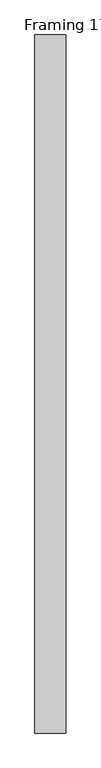
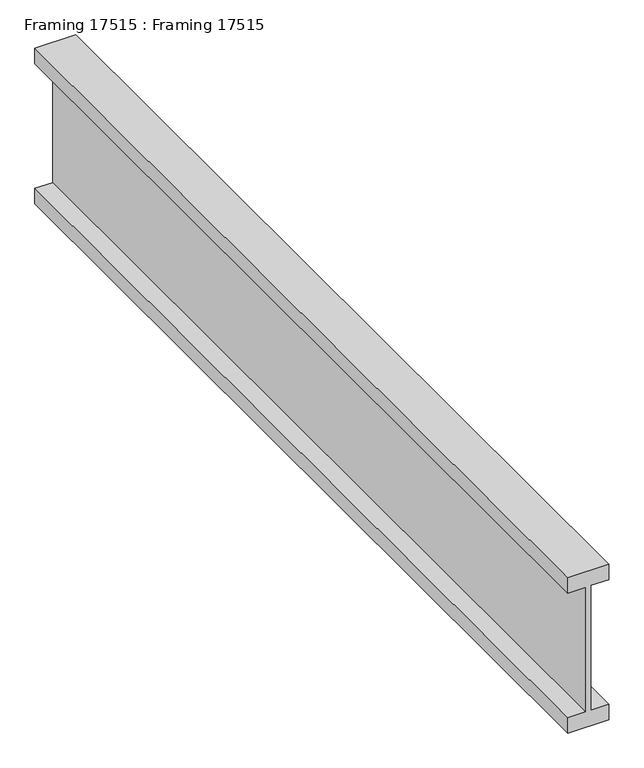
"""IFC4 building model written with IfcOpenShell, lengths in millimetres: proxy geometry, Framing 17515 : Framing 17515."""

import ifcopenshell
import ifcopenshell.guid

model = None  # the IFC model being written
_history = None  # IfcOwnerHistory: only IFC2X3 demands one
_inside = {}  # id of a spatial element -> (the spatial element, [elements in it])
_under = {}  # id of a project, library or spatial element -> (it, [spatial elements below it])
_declared = {}  # id of a project -> (the project, [libraries it declares])
_typed = {}  # id of a type object -> (the type object, [elements of that type])
_made_of = {}  # id of a material, layer set ... -> (it, [elements and type objects made of it])


def new_model(schema):
    """Start an empty IFC model of exactly this schema.

    Asked for "IFC4X3", IfcOpenShell would pick the latest addendum, in which some entities
    have other attributes; the version numbers below select the first issue.
    IFC2X3 requires an IfcOwnerHistory on every rooted entity: one is made here for all.
    """
    global model, _history
    if schema == "IFC4X3":
        model = ifcopenshell.file(schema_version=(4, 3, 0, 0))
    else:
        model = ifcopenshell.file(schema=schema)
    _inside.clear()
    _under.clear()
    _declared.clear()
    _typed.clear()
    _made_of.clear()
    _history = None
    if model.schema == "IFC2X3":
        org = make("IfcOrganization", Name="unknown")
        user = make(
            "IfcPersonAndOrganization",
            ThePerson=make("IfcPerson", FamilyName="unknown"),
            TheOrganization=org,
        )
        app = make(
            "IfcApplication",
            ApplicationDeveloper=org,
            Version="unknown",
            ApplicationFullName="unknown",
            ApplicationIdentifier="unknown",
        )
        _history = make(
            "IfcOwnerHistory",
            OwningUser=user,
            OwningApplication=app,
            ChangeAction="ADDED",
            CreationDate=0,
        )
    return model


def make(cls, **values):
    """One entity of the class cls with the attributes given. An attribute that is None is left unset."""
    return model.create_entity(
        cls, **{name: value for name, value in values.items() if value is not None}
    )


def rooted(cls, **values):
    """An entity with a GlobalId (a new one), such as an element, a storey or a relation."""
    return make(cls, GlobalId=ifcopenshell.guid.new(), OwnerHistory=_history, **values)


def si_unit(unit_type, name, prefix=None):
    """IfcSIUnit, for example si_unit("LENGTHUNIT", "METRE", prefix="MILLI")."""
    return make("IfcSIUnit", UnitType=unit_type, Prefix=prefix, Name=name)


def assignment(units):
    """IfcUnitAssignment: the units of a project."""
    return None if units is None else make("IfcUnitAssignment", Units=units)


def point(xyz):
    """IfcCartesianPoint."""
    return None if xyz is None else make("IfcCartesianPoint", Coordinates=xyz)


def direction(xyz):
    """IfcDirection."""
    return None if xyz is None else make("IfcDirection", DirectionRatios=xyz)


def frame(location, z_axis=None, x_axis=None):
    """IfcAxis2Placement3D, a coordinate frame: its origin and axes. An axis left out is left unset."""
    return make(
        "IfcAxis2Placement3D",
        Location=point(location),
        Axis=direction(z_axis),
        RefDirection=direction(x_axis),
    )


def origin():
    """The frame at (0, 0, 0) with its axes left unset."""
    return frame((0.0, 0.0, 0.0))


def place(relative_to, where):
    """IfcLocalPlacement: puts the frame where relative to a parent placement (None: the world)."""
    return make(
        "IfcLocalPlacement", PlacementRelTo=relative_to, RelativePlacement=where
    )


def context(
    kind, dimensions, precision=None, world=None, true_north=None, identifier=None
):
    """IfcGeometricRepresentationContext, for example the 3D "Model" context."""
    return make(
        "IfcGeometricRepresentationContext",
        ContextIdentifier=identifier,
        ContextType=kind,
        CoordinateSpaceDimension=dimensions,
        Precision=precision,
        WorldCoordinateSystem=world,
        TrueNorth=true_north,
    )


def project(units=None, contexts=None):
    """IfcProject with its units and contexts."""
    return rooted(
        "IfcProject",
        Name="project",
        RepresentationContexts=contexts,
        UnitsInContext=assignment(units),
    )


def spatial(cls, under=None, at=None, **own):
    """A site, building, storey or space (cls), placed at a placement, below another one or the project."""
    s = rooted(cls, ObjectPlacement=at, **own)
    if under is not None:
        _under.setdefault(under.id(), (under, []))[1].append(s)
    return s


def polyline(points):
    """IfcPolyline through the points."""
    return make("IfcPolyline", Points=[point(p) for p in points])


def outline(outer, holes=None, kind="AREA"):
    """IfcArbitraryClosedProfileDef: a profile drawn as a closed curve; with holes, ...WithVoids."""
    if holes is None:
        return make("IfcArbitraryClosedProfileDef", ProfileType=kind, OuterCurve=outer)
    return make(
        "IfcArbitraryProfileDefWithVoids",
        ProfileType=kind,
        OuterCurve=outer,
        InnerCurves=holes,
    )


def extrude(swept, where, along, depth):
    """IfcExtrudedAreaSolid: the profile swept, set in the frame where, extruded along a direction by depth."""
    return make(
        "IfcExtrudedAreaSolid",
        SweptArea=swept,
        Position=where,
        ExtrudedDirection=direction(along),
        Depth=depth,
    )


def shape(context_of_items, identifier, shape_type, items):
    """IfcShapeRepresentation: the items that make up one representation, for example the "Body"."""
    return make(
        "IfcShapeRepresentation",
        ContextOfItems=context_of_items,
        RepresentationIdentifier=identifier,
        RepresentationType=shape_type,
        Items=items,
    )


def source(mapping_origin, context_of_items, identifier, shape_type, items):
    """IfcRepresentationMap: a shape defined once, which mapped items show again and again."""
    return make(
        "IfcRepresentationMap",
        MappingOrigin=mapping_origin,
        MappedRepresentation=shape(context_of_items, identifier, shape_type, items),
    )


def transform(
    local_origin,
    x_axis=None,
    y_axis=None,
    z_axis=None,
    scale=None,
    scale2=None,
    scale3=None,
    uniform=True,
):
    """IfcCartesianTransformationOperator3D, or its non-uniform kind. x_axis, y_axis, z_axis: its Axis1, 2, 3."""
    if uniform:
        return make(
            "IfcCartesianTransformationOperator3D",
            Axis1=direction(x_axis),
            Axis2=direction(y_axis),
            LocalOrigin=point(local_origin),
            Scale=scale,
            Axis3=direction(z_axis),
        )
    return make(
        "IfcCartesianTransformationOperator3DnonUniform",
        Axis1=direction(x_axis),
        Axis2=direction(y_axis),
        LocalOrigin=point(local_origin),
        Scale=scale,
        Axis3=direction(z_axis),
        Scale2=scale2,
        Scale3=scale3,
    )


def mapped(mapping_source, mapping_target):
    """IfcMappedItem: shows the shape of a source again, moved by a transform."""
    return make(
        "IfcMappedItem", MappingSource=mapping_source, MappingTarget=mapping_target
    )


def made_of(thing, what):
    """Note that an element or type object is made of a material, layer set ...; save() writes the relation."""
    if what is not None:
        _made_of.setdefault(what.id(), (what, []))[1].append(thing)
    return thing


def element(
    cls,
    number,
    at=None,
    inside=None,
    cuts=None,
    type_object=None,
    material=None,
    context=None,
    identifier="Body",
    shape_type=None,
    held_by="IfcProductDefinitionShape",
    body=None,
    shapes=None,
    **own,
):
    """One element of the class cls, such as IfcWall. Its Tag is "e" and its number.

    at: its placement. inside: the storey or other place that contains it. cuts: it is an
    opening in that element (IfcRelVoidsElement). A single representation is given by context,
    identifier, shape_type and body (its items); several are given by shapes. held_by: the class
    of the entity that holds the representations. save() writes the other relations.
    """
    e = rooted(cls, Tag="e%d" % number, ObjectPlacement=at, **own)
    if body is not None:
        shapes = [shape(context, identifier, shape_type, body)]
    if shapes is not None:
        e.Representation = make(held_by, Representations=shapes)
    if inside is not None:
        _inside.setdefault(inside.id(), (inside, []))[1].append(e)
    if cuts is not None:
        rooted(
            "IfcRelVoidsElement", RelatingBuildingElement=cuts, RelatedOpeningElement=e
        )
    if type_object is not None:
        _typed.setdefault(type_object.id(), (type_object, []))[1].append(e)
    return made_of(e, material)


def aggregate(whole, parts):
    """IfcRelAggregates: a whole, such as a stair, and the parts it consists of."""
    return rooted("IfcRelAggregates", RelatingObject=whole, RelatedObjects=parts)


def save(model, path):
    """Write the relations noted so far, then the file.

    IfcRelAggregates (storeys below a building ...), IfcRelContainedInSpatialStructure (elements
    in a storey), IfcRelDefinesByType, IfcRelAssociatesMaterial and IfcRelDeclares: one each for
    every whole, place, type object, material and project.
    """
    for whole, parts in _under.values():
        aggregate(whole, parts)
    for where, things in _inside.values():
        rooted(
            "IfcRelContainedInSpatialStructure",
            RelatedElements=things,
            RelatingStructure=where,
        )
    for kind, things in _typed.values():
        rooted("IfcRelDefinesByType", RelatedObjects=things, RelatingType=kind)
    for what, things in _made_of.values():
        rooted("IfcRelAssociatesMaterial", RelatedObjects=things, RelatingMaterial=what)
    for by, libraries in _declared.values():
        rooted("IfcRelDeclares", RelatingContext=by, RelatedDefinitions=libraries)
    model.write(path)


def framing_17515_framing_17515_e96781f7(model_context):
    return source(origin(), model_context, "Body", "SweptSolid", [
        extrude(outline(polyline([(40077.771, 7689.895938), (39792.021, 7689.895938), (39792.021, 7651.002188), (39757.096, 7651.002188), (39757.096, 7739.902188), (39792.021, 7739.902188), (39792.021, 7701.008438), (40077.771, 7701.008438), (40077.771, 7739.902188), (40112.696, 7739.902188), (40112.696, 7651.002188), (40077.771, 7651.002188), (40077.771, 7689.895938)])), frame((0.0, -3747.9491938, 0.0), z_axis=(0.0, 1.0, 0.0), x_axis=(0.0, 0.0, 1.0)), (0.0, 0.0, 1.0), 2000.0),
    ])


if __name__ == "__main__":
    model = new_model("IFC4")
    model_context = context("Model", 3, world=origin())
    ifc_project = project(units=[si_unit("LENGTHUNIT", "METRE", prefix="MILLI")], contexts=[model_context])
    site = spatial("IfcSite", under=ifc_project)
    building = spatial("IfcBuilding", under=site)
    placement = place(None, origin())
    framing_17515_framing_17515_shape = framing_17515_framing_17515_e96781f7(model_context)
    element("IfcBuildingElementProxy", 1, Name="Framing 17515 : Framing 17515", ObjectType="Framing 17515 : Framing 17515", at=placement, inside=building, context=model_context, shape_type="MappedRepresentation", body=[
        mapped(framing_17515_framing_17515_shape, transform((0.0, 0.0, 0.0), x_axis=(1.0, 0.0, 0.0), y_axis=(0.0, 1.0, 0.0), z_axis=(0.0, 0.0, 1.0))),
    ])
    save(model, "model.ifc")

# Revit data of these elements
# Type "Framing 17515 : Framing 17515"
#   NameOverride = "Framing"
# Element 1 (IfcBuildingElementProxy, "Framing 17515 : Framing 17515")
#   Materials on its faces: "WOOD FRAMING (SEE STRUCT DWGS)"
# Materials
#   "WOOD FRAMING (SEE STRUCT DWGS)": class "Unassigned", colour RGB 224 188 168, transparency 0, Cost = 0
